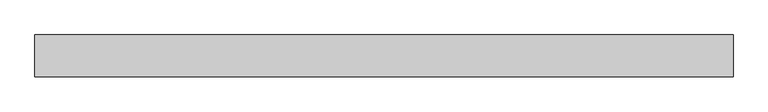
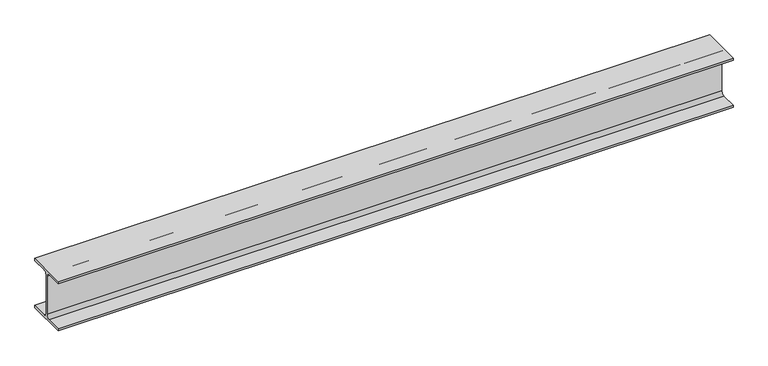
"""IFC4 building model written with IfcOpenShell, lengths in millimetres: beam geometry, 0912_Steel Framing_H-KSD3502 : H_SB_ASB_H-194x150x6x9."""

from ifc_helpers import new_model, si_unit, point, frame, frame_2d, origin, place, context, project, spatial, polyline, circle_curve, trimmed, segment, composite_curve, outline, extrude, source, transform, mapped, element, save


def beam_2ed9de13(model_context):
    return source(origin(), model_context, "Body", "SweptSolid", [
        extrude(outline(composite_curve([segment(polyline([(-75.0, -88.0), (-16.0, -88.0)]), True, "CONTINUOUS"), segment(trimmed(circle_curve(frame_2d((-16.0, -75.0)), 13.0), [point((-16.0, -88.0))], [point((-3.0, -75.0))], True, "CARTESIAN"), True, "CONTINUOUS"), segment(polyline([(-3.0, -75.0), (-3.0, 75.0)]), True, "CONTINUOUS"), segment(trimmed(circle_curve(frame_2d((-16.0, 75.0)), 13.0), [point((-3.0, 75.0))], [point((-16.0, 88.0))], True, "CARTESIAN"), True, "CONTINUOUS"), segment(polyline([(-16.0, 88.0), (-75.0, 88.0), (-75.0, 97.0), (75.0, 97.0), (75.0, 88.0), (16.0, 88.0)]), True, "CONTINUOUS"), segment(trimmed(circle_curve(frame_2d((16.0, 75.0)), 13.0), [point((16.0, 88.0))], [point((3.0, 75.0))], True, "CARTESIAN"), True, "CONTINUOUS"), segment(polyline([(3.0, 75.0), (3.0, -75.0)]), True, "CONTINUOUS"), segment(trimmed(circle_curve(frame_2d((16.0, -75.0)), 13.0), [point((3.0, -75.0))], [point((16.0, -88.0))], True, "CARTESIAN"), True, "CONTINUOUS"), segment(polyline([(16.0, -88.0), (75.0, -88.0), (75.0, -97.0), (-75.0, -97.0), (-75.0, -88.0)]), True, "CONTINUOUS")], self_intersect=False)), frame((-1253.7727018, 0.0, 0.0), z_axis=(1.0, 0.0, 0.0), x_axis=(0.0, 1.0, 0.0)), (0.0, 0.0, 1.0), 2507.5454037),
    ])


if __name__ == "__main__":
    model = new_model("IFC4")
    model_context = context("Model", 3, world=origin())
    ifc_project = project(units=[si_unit("LENGTHUNIT", "METRE", prefix="MILLI")], contexts=[model_context])
    site = spatial("IfcSite", under=ifc_project)
    building = spatial("IfcBuilding", under=site)
    placement = place(None, origin())
    beam_shape = beam_2ed9de13(model_context)
    element("IfcBeam", 1, ObjectType="0912_Steel Framing_H-KSD3502 : H_SB_ASB_H-194x150x6x9", at=placement, inside=building, context=model_context, shape_type="MappedRepresentation", body=[
        mapped(beam_shape, transform((0.0, 0.0, 0.0), x_axis=(1.0, 0.0, 0.0), y_axis=(0.0, 1.0, 0.0), z_axis=(0.0, 0.0, 1.0))),
    ])
    save(model, "model.ifc")

# Revit data of these elements
# Type "0912_Steel Framing_H-KSD3502 : H_SB_ASB_H-194x150x6x9"
#   H_WM Code_1 = "S01AA002-00001 | Main Steel Structure Fabrication Work | Shelter/Building | Medium Steel - Standard (90KG/M>Weight≥30KG/M) | Material: (   )"
#   H_WM Code_2 = "S03AA028-00001 | Main Steel Structure Erection Work | Shelter/Building | Medium Steel (90KG/M>Weight≥30KG/M) | Material: (   )"
#   H_WM Code_3 = "S01AA010-00001 | Main Steel Structure Fabrication Work | Shelter/Building | Steel Painting/Coating | for Non-Fireproofed Steel Surface, Surface Preparation, Primer, Second & Final Coat | Material: (   )"
#   H_Q'ty Cal Type Tag = "SB-Q2"
#   Width = 15.0 cm
#   Web Thickness = 0.6 cm
#   Web Fillet = 1.3 cm
#   Warping Constant = 43316.0 cm⁶
#   W = 0
#   Torsional Moment of Inertia = 8.622 cm⁴
#   Section Area = 39.01 cm²
#   Plastic Modulus weak axis = 104.0 cm³
#   Plastic Modulus strong axis = 309.0 cm³
#   Perimeter = 0.95 m²/m
#   Nominal Weight = 30.60 kgf/m
#   Moment of Inertia weak axis = 507.00 cm⁴
#   Moment of Inertia strong axis = 2690.00 cm⁴
#   Height = 19.4 cm
#   Flange Thickness = 0.9 cm
#   Elastic Modulus weak axis = 67.6 cm³
#   Elastic Modulus strong axis = 277.0 cm³
#   Centroid Vertical = 9.7 cm
#   Centroid Horizontal = 7.5 cm
#   Ix = 26900000
#   Length [instance default] = 1.5240 m
#   Zx = 309000
#   b = 0.1500 m
#   h = 0.1940 m
#   r = 0.0130 m
#   s = 0.0060 m
#   t = 0.0090 m
#   A = 0.003901 m²
#   Structural Material [instance default] = Steel, 45-345
#   Assembly Code = ""
# Element 1 (IfcBeam, "0912_Steel Framing_H-KSD3502 : H_SB_ASB_H-194x150x6x9")
#   Structural Material = none
# Materials
#   "Steel, 45-345": class "Metal", colour RGB 189 187 185, transparency 0, Description = "Steel 345 MPa", Cost = 0
